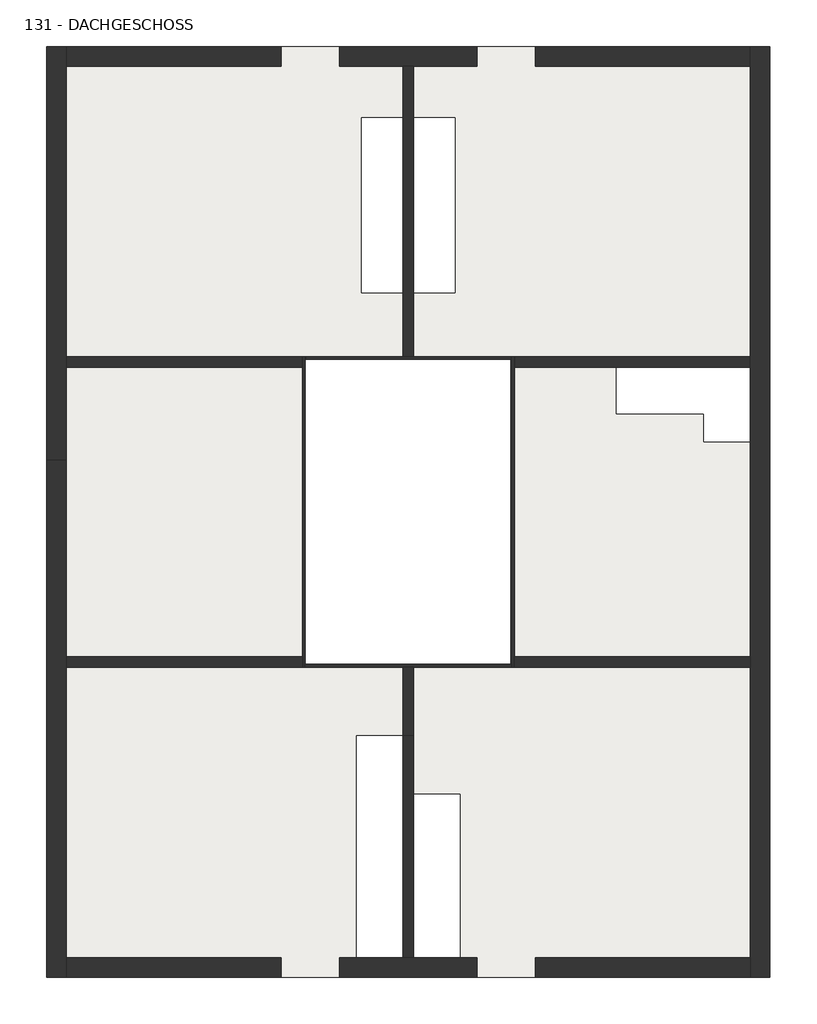
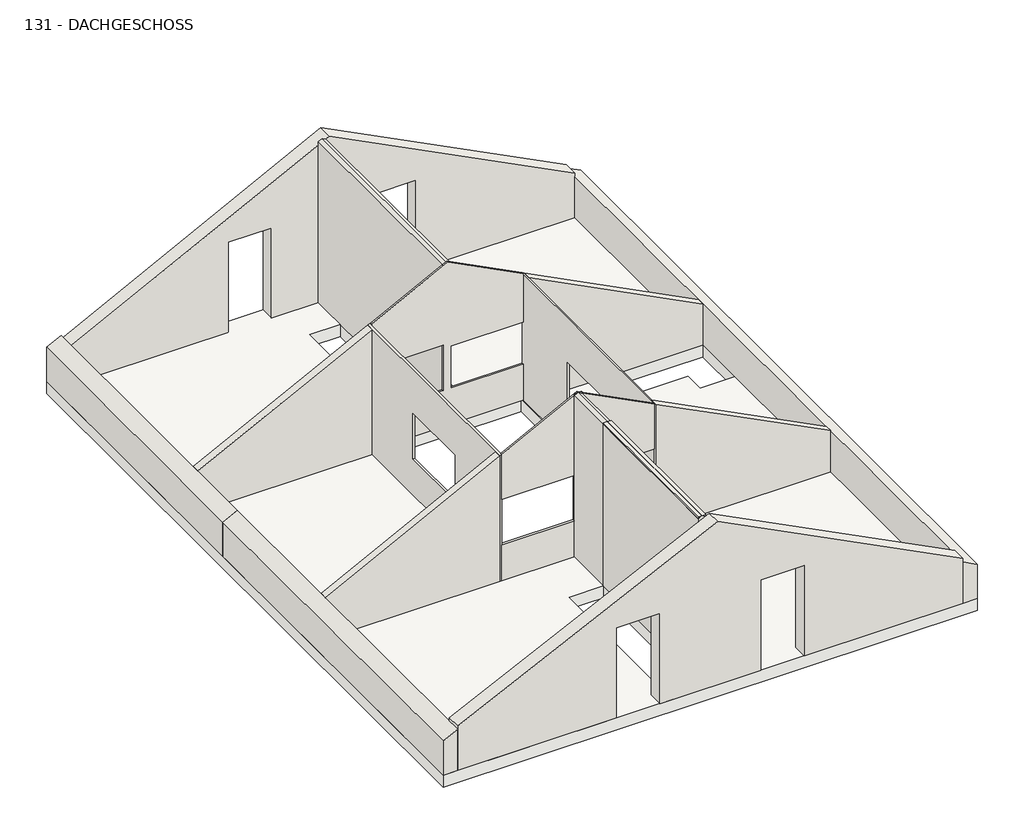
# One storey: 16 walls, 1 slab.
"""IFC4 building model written with IfcOpenShell, lengths in millimetres."""

import ifcopenshell
import ifcopenshell.guid

model = None  # the IFC model being written
_history = None  # IfcOwnerHistory: only IFC2X3 demands one
_inside = {}  # id of a spatial element -> (the spatial element, [elements in it])
_under = {}  # id of a project, library or spatial element -> (it, [spatial elements below it])
_declared = {}  # id of a project -> (the project, [libraries it declares])
_typed = {}  # id of a type object -> (the type object, [elements of that type])
_made_of = {}  # id of a material, layer set ... -> (it, [elements and type objects made of it])


def new_model(schema):
    """Start an empty IFC model of exactly this schema.

    Asked for "IFC4X3", IfcOpenShell would pick the latest addendum, in which some entities
    have other attributes; the version numbers below select the first issue.
    IFC2X3 requires an IfcOwnerHistory on every rooted entity: one is made here for all.
    """
    global model, _history
    if schema == "IFC4X3":
        model = ifcopenshell.file(schema_version=(4, 3, 0, 0))
    else:
        model = ifcopenshell.file(schema=schema)
    _inside.clear()
    _under.clear()
    _declared.clear()
    _typed.clear()
    _made_of.clear()
    _history = None
    if model.schema == "IFC2X3":
        org = make("IfcOrganization", Name="unknown")
        user = make(
            "IfcPersonAndOrganization",
            ThePerson=make("IfcPerson", FamilyName="unknown"),
            TheOrganization=org,
        )
        app = make(
            "IfcApplication",
            ApplicationDeveloper=org,
            Version="unknown",
            ApplicationFullName="unknown",
            ApplicationIdentifier="unknown",
        )
        _history = make(
            "IfcOwnerHistory",
            OwningUser=user,
            OwningApplication=app,
            ChangeAction="ADDED",
            CreationDate=0,
        )
    return model


def make(cls, **values):
    """One entity of the class cls with the attributes given. An attribute that is None is left unset."""
    return model.create_entity(
        cls, **{name: value for name, value in values.items() if value is not None}
    )


def rooted(cls, **values):
    """An entity with a GlobalId (a new one), such as an element, a storey or a relation."""
    return make(cls, GlobalId=ifcopenshell.guid.new(), OwnerHistory=_history, **values)


def si_unit(unit_type, name, prefix=None):
    """IfcSIUnit, for example si_unit("LENGTHUNIT", "METRE", prefix="MILLI")."""
    return make("IfcSIUnit", UnitType=unit_type, Prefix=prefix, Name=name)


def assignment(units):
    """IfcUnitAssignment: the units of a project."""
    return None if units is None else make("IfcUnitAssignment", Units=units)


def point(xyz):
    """IfcCartesianPoint."""
    return None if xyz is None else make("IfcCartesianPoint", Coordinates=xyz)


def direction(xyz):
    """IfcDirection."""
    return None if xyz is None else make("IfcDirection", DirectionRatios=xyz)


def frame(location, z_axis=None, x_axis=None):
    """IfcAxis2Placement3D, a coordinate frame: its origin and axes. An axis left out is left unset."""
    return make(
        "IfcAxis2Placement3D",
        Location=point(location),
        Axis=direction(z_axis),
        RefDirection=direction(x_axis),
    )


def origin():
    """The frame at (0, 0, 0) with its axes left unset."""
    return frame((0.0, 0.0, 0.0))


def place(relative_to, where):
    """IfcLocalPlacement: puts the frame where relative to a parent placement (None: the world)."""
    return make(
        "IfcLocalPlacement", PlacementRelTo=relative_to, RelativePlacement=where
    )


def context(
    kind, dimensions, precision=None, world=None, true_north=None, identifier=None
):
    """IfcGeometricRepresentationContext, for example the 3D "Model" context."""
    return make(
        "IfcGeometricRepresentationContext",
        ContextIdentifier=identifier,
        ContextType=kind,
        CoordinateSpaceDimension=dimensions,
        Precision=precision,
        WorldCoordinateSystem=world,
        TrueNorth=true_north,
    )


def project(units=None, contexts=None):
    """IfcProject with its units and contexts."""
    return rooted(
        "IfcProject",
        Name="project",
        RepresentationContexts=contexts,
        UnitsInContext=assignment(units),
    )


def spatial(cls, under=None, at=None, **own):
    """A site, building, storey or space (cls), placed at a placement, below another one or the project."""
    s = rooted(cls, ObjectPlacement=at, **own)
    if under is not None:
        _under.setdefault(under.id(), (under, []))[1].append(s)
    return s


def polyline(points):
    """IfcPolyline through the points."""
    return make("IfcPolyline", Points=[point(p) for p in points])


def outline(outer, holes=None, kind="AREA"):
    """IfcArbitraryClosedProfileDef: a profile drawn as a closed curve; with holes, ...WithVoids."""
    if holes is None:
        return make("IfcArbitraryClosedProfileDef", ProfileType=kind, OuterCurve=outer)
    return make(
        "IfcArbitraryProfileDefWithVoids",
        ProfileType=kind,
        OuterCurve=outer,
        InnerCurves=holes,
    )


def extrude(swept, where, along, depth):
    """IfcExtrudedAreaSolid: the profile swept, set in the frame where, extruded along a direction by depth."""
    return make(
        "IfcExtrudedAreaSolid",
        SweptArea=swept,
        Position=where,
        ExtrudedDirection=direction(along),
        Depth=depth,
    )


def faces_of(points, faces, orient=None, outer=None):
    """IfcFace entities. A face is a list of loops; a loop is a list of indices into points, from 0.

    orient and outer hold one flag for each loop. By default every Orientation is true, the
    first loop of a face is its IfcFaceOuterBound and the others are IfcFaceBound.
    """
    made = []
    for i, loops in enumerate(faces):
        bounds = []
        for j, loop in enumerate(loops):
            is_outer = j == 0 if outer is None else outer[i][j]
            bounds.append(
                make(
                    "IfcFaceOuterBound" if is_outer else "IfcFaceBound",
                    Bound=make("IfcPolyLoop", Polygon=[points[k] for k in loop]),
                    Orientation=True if orient is None else orient[i][j],
                )
            )
        made.append(make("IfcFace", Bounds=bounds))
    return made


def faceted_brep(points, faces, orient=None, outer=None, voids=None):
    """IfcFacetedBrep: a solid bounded by flat faces; with voids (closed shells), ...WithVoids."""
    shared = [point(p) for p in points]
    hull = make("IfcClosedShell", CfsFaces=faces_of(shared, faces, orient, outer))
    if voids is None:
        return make("IfcFacetedBrep", Outer=hull)
    return make(
        "IfcFacetedBrepWithVoids",
        Outer=hull,
        Voids=[
            make(cls, CfsFaces=faces_of(shared, fs, o, b)) for cls, fs, o, b in voids
        ],
    )


def shape(context_of_items, identifier, shape_type, items):
    """IfcShapeRepresentation: the items that make up one representation, for example the "Body"."""
    return make(
        "IfcShapeRepresentation",
        ContextOfItems=context_of_items,
        RepresentationIdentifier=identifier,
        RepresentationType=shape_type,
        Items=items,
    )


def source(mapping_origin, context_of_items, identifier, shape_type, items):
    """IfcRepresentationMap: a shape defined once, which mapped items show again and again."""
    return make(
        "IfcRepresentationMap",
        MappingOrigin=mapping_origin,
        MappedRepresentation=shape(context_of_items, identifier, shape_type, items),
    )


def transform(
    local_origin,
    x_axis=None,
    y_axis=None,
    z_axis=None,
    scale=None,
    scale2=None,
    scale3=None,
    uniform=True,
):
    """IfcCartesianTransformationOperator3D, or its non-uniform kind. x_axis, y_axis, z_axis: its Axis1, 2, 3."""
    if uniform:
        return make(
            "IfcCartesianTransformationOperator3D",
            Axis1=direction(x_axis),
            Axis2=direction(y_axis),
            LocalOrigin=point(local_origin),
            Scale=scale,
            Axis3=direction(z_axis),
        )
    return make(
        "IfcCartesianTransformationOperator3DnonUniform",
        Axis1=direction(x_axis),
        Axis2=direction(y_axis),
        LocalOrigin=point(local_origin),
        Scale=scale,
        Axis3=direction(z_axis),
        Scale2=scale2,
        Scale3=scale3,
    )


def mapped(mapping_source, mapping_target):
    """IfcMappedItem: shows the shape of a source again, moved by a transform."""
    return make(
        "IfcMappedItem", MappingSource=mapping_source, MappingTarget=mapping_target
    )


def made_of(thing, what):
    """Note that an element or type object is made of a material, layer set ...; save() writes the relation."""
    if what is not None:
        _made_of.setdefault(what.id(), (what, []))[1].append(thing)
    return thing


def element(
    cls,
    number,
    at=None,
    inside=None,
    cuts=None,
    type_object=None,
    material=None,
    context=None,
    identifier="Body",
    shape_type=None,
    held_by="IfcProductDefinitionShape",
    body=None,
    shapes=None,
    **own,
):
    """One element of the class cls, such as IfcWall. Its Tag is "e" and its number.

    at: its placement. inside: the storey or other place that contains it. cuts: it is an
    opening in that element (IfcRelVoidsElement). A single representation is given by context,
    identifier, shape_type and body (its items); several are given by shapes. held_by: the class
    of the entity that holds the representations. save() writes the other relations.
    """
    e = rooted(cls, Tag="e%d" % number, ObjectPlacement=at, **own)
    if body is not None:
        shapes = [shape(context, identifier, shape_type, body)]
    if shapes is not None:
        e.Representation = make(held_by, Representations=shapes)
    if inside is not None:
        _inside.setdefault(inside.id(), (inside, []))[1].append(e)
    if cuts is not None:
        rooted(
            "IfcRelVoidsElement", RelatingBuildingElement=cuts, RelatedOpeningElement=e
        )
    if type_object is not None:
        _typed.setdefault(type_object.id(), (type_object, []))[1].append(e)
    return made_of(e, material)


def aggregate(whole, parts):
    """IfcRelAggregates: a whole, such as a stair, and the parts it consists of."""
    return rooted("IfcRelAggregates", RelatingObject=whole, RelatedObjects=parts)


def save(model, path):
    """Write the relations noted so far, then the file.

    IfcRelAggregates (storeys below a building ...), IfcRelContainedInSpatialStructure (elements
    in a storey), IfcRelDefinesByType, IfcRelAssociatesMaterial and IfcRelDeclares: one each for
    every whole, place, type object, material and project.
    """
    for whole, parts in _under.values():
        aggregate(whole, parts)
    for where, things in _inside.values():
        rooted(
            "IfcRelContainedInSpatialStructure",
            RelatedElements=things,
            RelatingStructure=where,
        )
    for kind, things in _typed.values():
        rooted("IfcRelDefinesByType", RelatedObjects=things, RelatingType=kind)
    for what, things in _made_of.values():
        rooted("IfcRelAssociatesMaterial", RelatedObjects=things, RelatingMaterial=what)
    for by, libraries in _declared.values():
        rooted("IfcRelDeclares", RelatingContext=by, RelatedDefinitions=libraries)
    model.write(path)


def slab_52cff1b9(model_context):
    return source(origin(), model_context, "Body", "SweptSolid", [
        extrude(outline(polyline([(172797.7593015, 28481.9343946), (158797.7593015, 28481.9343946), (158797.7593015, 46484.7962965), (172797.7593015, 46484.7962965), (172797.7593015, 28481.9343946)]), holes=[polyline([(167772.7593015, 40484.7962965), (163772.7593015, 40484.7962965), (163772.7593015, 34484.7962965), (167772.7593015, 34484.7962965), (167772.7593015, 40484.7962965)]), polyline([(165697.7593015, 33159.7962965), (164797.7593015, 33159.7962965), (164797.7593015, 28861.9343946), (165697.7593015, 28861.9343946), (165697.7593015, 33159.7962965)]), polyline([(165897.7593015, 32021.9343946), (165897.7593015, 29779.7962965), (165897.7593015, 28861.9343946), (166797.7593015, 28861.9343946), (166797.7593015, 32021.9343946), (165897.7593015, 32021.9343946)]), polyline([(171517.7593015, 38844.7962965), (172417.7593015, 38844.7962965), (172417.7593015, 40284.7962965), (169822.7593015, 40284.7962965), (169822.7593015, 39384.7962965), (171517.7593015, 39384.7962965), (171517.7593015, 38844.7962965)]), polyline([(165897.7593015, 45104.7962965), (165897.7593015, 41724.7962965), (166697.7593015, 41724.7962965), (166697.7593015, 45104.7962965), (165897.7593015, 45104.7962965)]), polyline([(164897.7593015, 41724.7962965), (165697.7593015, 41724.7962965), (165697.7593015, 45104.7962965), (164897.7593015, 45104.7962965), (164897.7593015, 41724.7962965)])]), frame((0.0, 0.0, 5830.0), z_axis=(0.0, 0.0, 1.0), x_axis=(1.0, 0.0, 0.0)), (0.0, 0.0, 1.0), 330.0),
    ])


model = new_model("IFC4")

# Units and contexts
model_context = context("Model", 3, world=origin())
ifc_project = project(units=[si_unit("LENGTHUNIT", "METRE", prefix="MILLI")], contexts=[model_context])

# Site, building, storey
site = spatial("IfcSite", under=ifc_project)
building = spatial("IfcBuilding", under=site)
storey = spatial("IfcBuildingStorey", under=building, Name="131 - DACHGESCHOSS", Elevation=5650.0)

# Slab
placement = place(None, origin())
slab_shape = slab_52cff1b9(model_context)
element("IfcSlab", 1, ObjectType="Holzdecke 142136 : Holzdecke 142136", at=placement, inside=storey, context=model_context, shape_type="MappedRepresentation", body=[
    mapped(slab_shape, transform((-157297.7593015, -26934.7962965, 0.0), x_axis=(1.0, 0.0, 0.0), y_axis=(0.0, 1.0, 0.0), z_axis=(0.0, 0.0, 1.0))),
])

# Walls
element("IfcWall", 2, ObjectType="Holzwand", at=placement, inside=storey, context=model_context, shape_type="SweptSolid", body=[
    extrude(outline(polyline([(6160.0, 10550.0), (6160.0, 15120.0), (7303.6196708, 15120.0), (9632.150975, 10550.0), (6160.0, 10550.0)])), frame((0.0, 7550.0, 0.0), z_axis=(0.0, 1.0, 0.0), x_axis=(0.0, 0.0, 1.0)), (0.0, 0.0, 1.0), 200.0),
])
element("IfcWall", 3, ObjectType="Holzwand:1197", at=placement, inside=storey, context=model_context, shape_type="SweptSolid", body=[
    extrude(outline(polyline([(6160.0, 1880.0), (6160.0, 6450.0), (9632.150975, 6450.0), (7303.6196708, 1880.0), (6160.0, 1880.0)])), frame((0.0, 7550.0, 0.0), z_axis=(0.0, 1.0, 0.0), x_axis=(0.0, 0.0, 1.0)), (0.0, 0.0, 1.0), 200.0),
])
element("IfcWall", 4, ObjectType="Holzwand:1195", at=placement, inside=storey, context=model_context, shape_type="SweptSolid", body=[
    extrude(outline(polyline([(6160.0, 10550.0), (6160.0, 15120.0), (7303.6196708, 15120.0), (9632.150975, 10550.0), (6160.0, 10550.0)])), frame((0.0, 13350.0, 0.0), z_axis=(0.0, 1.0, 0.0), x_axis=(0.0, 0.0, 1.0)), (0.0, 0.0, 1.0), 200.0),
])
element("IfcWall", 5, ObjectType="Holzwand:1193", at=placement, inside=storey, context=model_context, shape_type="SweptSolid", body=[
    extrude(outline(polyline([(6160.0, 1880.0), (6160.0, 6450.0), (9632.150975, 6450.0), (7303.6196708, 1880.0), (6160.0, 1880.0)])), frame((0.0, 13350.0, 0.0), z_axis=(0.0, 1.0, 0.0), x_axis=(0.0, 0.0, 1.0)), (0.0, 0.0, 1.0), 200.0),
])
element("IfcWall", 6, ObjectType=" ", at=placement, inside=storey, context=model_context, shape_type="Brep", body=[
    faceted_brep([(6500.0, 7550.0, 6160.0), (6500.0, 7600.0, 6160.0), (6500.0, 13550.0, 6160.0), (6500.0, 13550.0, 9657.6272475), (6500.0, 7600.0, 9657.6272475), (6500.0, 7550.0, 9657.6272475), (6500.0, 7550.0, 8420.0), (6500.0, 7550.0, 7160.0), (6500.0, 11500.0, 8420.0), (6500.0, 11500.0, 7160.0), (6500.0, 9600.0, 7160.0), (6500.0, 9600.0, 8420.0), (6450.0, 13550.0, 6160.0), (6450.0, 7550.0, 6160.0), (6450.0, 7550.0, 9632.150975), (6450.0, 13550.0, 9632.150975), (6450.0, 11500.0, 7160.0), (6450.0, 11500.0, 8420.0), (6450.0, 9600.0, 8420.0), (6450.0, 9600.0, 7160.0)], [[[0, 1, 2, 3, 4, 5, 6, 7], [8, 9, 10, 11]], [[12, 13, 14, 15], [16, 17, 18, 19]], [[2, 1, 0, 13, 12]], [[5, 4, 3, 15, 14]], [[8, 17, 16, 9]], [[17, 8, 11, 18]], [[18, 11, 10, 19]], [[9, 16, 19, 10]], [[0, 7, 6, 5, 14, 13]], [[3, 2, 12, 15]]]),
])
element("IfcWall", 7, ObjectType=" :1188", at=placement, inside=storey, context=model_context, shape_type="Brep", body=[
    faceted_brep([(10500.0, 7600.0, 6160.0), (6500.0, 7600.0, 6160.0), (6500.0, 7600.0, 7160.0), (8400.0, 7600.0, 7160.0), (8400.0, 7600.0, 8420.0), (6500.0, 7600.0, 8420.0), (6500.0, 7600.0, 9657.6272475), (8500.0, 7600.0, 10676.6781465), (10500.0, 7600.0, 9657.6272475), (10500.0, 7600.0, 8420.0), (8607.9636779, 7600.0, 8420.0), (8607.9636779, 7600.0, 7160.0), (10500.0, 7600.0, 7160.0), (6500.0, 7550.0, 6160.0), (10500.0, 7550.0, 6160.0), (10500.0, 7550.0, 7160.0), (8607.9636779, 7550.0, 7160.0), (8607.9636779, 7550.0, 8420.0), (10500.0, 7550.0, 8420.0), (10500.0, 7550.0, 9657.6272475), (8600.0, 7550.0, 10625.7256015), (8600.0, 7550.0, 10676.6781465), (8400.0, 7550.0, 10676.6781465), (8400.0, 7550.0, 10625.7256015), (6500.0, 7550.0, 9657.6272475), (6500.0, 7550.0, 8420.0), (8400.0, 7550.0, 8420.0), (8400.0, 7550.0, 7160.0), (6500.0, 7550.0, 7160.0), (8500.0, 7550.4030929, 10676.6781465)], [[[0, 1, 2, 3, 4, 5, 6, 7, 8, 9, 10, 11, 12]], [[13, 14, 15, 16, 17, 18, 19, 20, 21, 22, 23, 24, 25, 26, 27, 28]], [[1, 0, 14, 13]], [[22, 21, 29]], [[29, 20, 19, 8, 7]], [[20, 29, 21]], [[29, 7, 6, 24, 23]], [[29, 23, 22]], [[4, 26, 25, 5]], [[26, 4, 3, 27]], [[27, 3, 2, 28]], [[10, 17, 16, 11]], [[17, 10, 9, 18]], [[11, 16, 15, 12]], [[8, 19, 18, 9]], [[14, 0, 12, 15]], [[24, 6, 5, 25]], [[1, 13, 28, 2]]]),
])
element("IfcWall", 8, ObjectType=" :1186", at=placement, inside=storey, context=model_context, shape_type="Brep", body=[
    faceted_brep([(10500.0, 13550.0, 6160.0), (10500.0, 13500.0, 6160.0), (10500.0, 7600.0, 6160.0), (10500.0, 7550.0, 6160.0), (10500.0, 7550.0, 7160.0), (10500.0, 7550.0, 8420.0), (10500.0, 7550.0, 9657.6272475), (10500.0, 7600.0, 9657.6272475), (10500.0, 13550.0, 9657.6272475), (10500.0, 13550.0, 8320.0), (10500.0, 13550.0, 7160.0), (10500.0, 9600.0, 8420.0), (10500.0, 9600.0, 7160.0), (10500.0, 11500.0, 7160.0), (10500.0, 11500.0, 8420.0), (10550.0, 7550.0, 6160.0), (10550.0, 13550.0, 6160.0), (10550.0, 13550.0, 9632.150975), (10550.0, 7550.0, 9632.150975), (10550.0, 9600.0, 7160.0), (10550.0, 9600.0, 8420.0), (10550.0, 11500.0, 8420.0), (10550.0, 11500.0, 7160.0)], [[[0, 1, 2, 3, 4, 5, 6, 7, 8, 9, 10], [11, 12, 13, 14]], [[15, 16, 17, 18], [19, 20, 21, 22]], [[3, 2, 1, 0, 16, 15]], [[8, 7, 6, 18, 17]], [[19, 12, 11, 20]], [[20, 11, 14, 21]], [[21, 14, 13, 22]], [[12, 19, 22, 13]], [[6, 5, 4, 3, 15, 18]], [[0, 10, 9, 8, 17, 16]]]),
])
element("IfcWall", 9, ObjectType="Holzwand:1184", at=placement, inside=storey, context=model_context, shape_type="SweptSolid", body=[
    extrude(outline(polyline([(6160.0, 8400.0), (6160.0, 8600.0), (10625.7256015, 8600.0), (10676.6781465, 8500.0), (10625.7256015, 8400.0), (6160.0, 8400.0)])), frame((0.0, 1927.1380981, 0.0), z_axis=(0.0, 1.0, 0.0), x_axis=(0.0, 0.0, 1.0)), (0.0, 0.0, 1.0), 4297.8619019),
])
element("IfcWall", 10, ObjectType="Holzwand:1180", at=placement, inside=storey, context=model_context, shape_type="SweptSolid", body=[
    extrude(outline(polyline([(6160.0, 8400.0), (6160.0, 8600.0), (10625.7256015, 8600.0), (10676.6781465, 8500.0), (10625.7256015, 8400.0), (6160.0, 8400.0)])), frame((0.0, 13550.0, 0.0), z_axis=(0.0, 1.0, 0.0), x_axis=(0.0, 0.0, 1.0)), (0.0, 0.0, 1.0), 5620.0),
])
element("IfcWall", 11, ObjectType="Holzwand:1178", at=placement, inside=storey, context=model_context, shape_type="Brep", body=[
    faceted_brep([(8600.0, 1927.541191, 6160.0), (8600.0, 7550.0, 6160.0), (8600.0, 7550.0, 10625.7256015), (8600.0, 6225.0, 10625.7256015), (8600.0, 6225.0, 10676.6781465), (8600.0, 1927.541191, 10676.6781465), (8400.0, 7550.0, 6160.0), (8400.0, 1927.541191, 6160.0), (8400.0, 1927.541191, 10676.6781465), (8400.0, 6225.0, 10676.6781465), (8400.0, 6225.0, 10625.7256015), (8400.0, 7550.0, 10625.7256015), (8500.0, 6225.0, 10676.6781465), (8500.0, 7550.0, 10676.6781465)], [[[0, 1, 2, 3, 4, 5]], [[6, 7, 8, 9, 10, 11]], [[1, 0, 7, 6]], [[8, 5, 4, 12, 9]], [[0, 5, 8, 7]], [[12, 3, 2, 13]], [[3, 12, 4]], [[12, 10, 9]], [[10, 12, 13, 11]], [[1, 6, 11, 13, 2]]]),
])
element("IfcWall", 12, ObjectType=" :1190", at=placement, inside=storey, context=model_context, shape_type="Brep", body=[
    faceted_brep([(6525.0, 13500.0, 6160.0), (10500.0, 13500.0, 6160.0), (10500.0, 13500.0, 7160.0), (8600.0, 13500.0, 7160.0), (8600.0, 13500.0, 8320.0), (10500.0, 13500.0, 8320.0), (10500.0, 13500.0, 9670.3653837), (8525.0, 13500.0, 10676.6781465), (6525.0, 13500.0, 9657.6272475), (6525.0, 13500.0, 8420.0), (8400.0, 13500.0, 8420.0), (8400.0, 13500.0, 7160.0), (6525.0, 13500.0, 7160.0), (10500.0, 13550.0, 6160.0), (6525.0, 13550.0, 6160.0), (6525.0, 13550.0, 7160.0), (8400.0, 13550.0, 7160.0), (8400.0, 13550.0, 8420.0), (6525.0, 13550.0, 8420.0), (6525.0, 13550.0, 9657.6272475), (8525.0, 13550.0, 10676.6781465), (10500.0, 13550.0, 9670.3653837), (10500.0, 13550.0, 9657.6272475), (10500.0, 13550.0, 8320.0), (8600.0, 13550.0, 8320.0), (8600.0, 13550.0, 7160.0), (10500.0, 13550.0, 7160.0)], [[[0, 1, 2, 3, 4, 5, 6, 7, 8, 9, 10, 11, 12]], [[13, 14, 15, 16, 17, 18, 19, 20, 21, 22, 23, 24, 25, 26]], [[1, 0, 14, 13]], [[7, 6, 21, 20]], [[8, 7, 20, 19]], [[8, 19, 18, 9]], [[14, 0, 12, 15]], [[10, 17, 16, 11]], [[17, 10, 9, 18]], [[11, 16, 15, 12]], [[4, 24, 23, 5]], [[24, 4, 3, 25]], [[25, 3, 2, 26]], [[21, 6, 5, 23, 22]], [[1, 13, 26, 2]]]),
])
element("IfcWall", 13, ObjectType="1141 Aussenwand", at=placement, inside=storey, context=model_context, shape_type="Brep", body=[
    faceted_brep([(1880.0, 1547.1380981, 6160.0), (1880.0, 1927.1380981, 6160.0), (1880.0, 11550.0, 6160.0), (1880.0, 11550.0, 7303.6196708), (1880.0, 1547.1380981, 7303.6196708), (1500.0, 11550.0, 6160.0), (1500.0, 1547.1380981, 6160.0), (1500.0, 1547.1380981, 7110.0), (1500.0, 11550.0, 7110.0)], [[[0, 1, 2, 3, 4]], [[5, 6, 7, 8]], [[2, 1, 0, 6, 5]], [[3, 2, 5, 8]], [[4, 3, 8, 7]], [[0, 4, 7, 6]]]),
])
element("IfcWall", 14, ObjectType="1141 Aussenwand", at=placement, inside=storey, context=model_context, shape_type="Brep", body=[
    faceted_brep([(15120.0, 19550.0, 6160.0), (15120.0, 19170.0, 6160.0), (15120.0, 1927.1380981, 6160.0), (15120.0, 1547.1380981, 6160.0), (15120.0, 1547.1380981, 7303.6196708), (15120.0, 19550.0, 7303.6196708), (15500.0, 1547.1380981, 6160.0), (15500.0, 19550.0, 6160.0), (15500.0, 19550.0, 7110.0), (15500.0, 1547.1380981, 7110.0)], [[[0, 1, 2, 3, 4, 5]], [[6, 7, 8, 9]], [[3, 2, 1, 0, 7, 6]], [[5, 4, 9, 8]], [[4, 3, 6, 9]], [[0, 5, 8, 7]]]),
])
element("IfcWall", 15, ObjectType="1141 Aussenwand", at=placement, inside=storey, context=model_context, shape_type="Brep", body=[
    faceted_brep([(1880.0, 11550.0, 6160.0), (1880.0, 19170.0, 6160.0), (1880.0, 19550.0, 6160.0), (1880.0, 19550.0, 7206.8098354), (1880.0, 19550.0, 7303.6196708), (1880.0, 11550.0, 7303.6196708), (1500.0, 19550.0, 6160.0), (1500.0, 11550.0, 6160.0), (1500.0, 11550.0, 7110.0), (1500.0, 19550.0, 7110.0)], [[[0, 1, 2, 3, 4, 5]], [[6, 7, 8, 9]], [[2, 1, 0, 7, 6]], [[0, 5, 8, 7]], [[5, 4, 9, 8]], [[4, 3, 2, 6, 9]]]),
])
element("IfcWall", 16, ObjectType="1141 Aussenwand", at=placement, inside=storey, context=model_context, shape_type="Brep", body=[
    faceted_brep([(1880.0, 1927.1380981, 7395.1741151), (8690.0, 1927.1380981, 10676.6781465), (15120.0, 1927.1380981, 7400.4295062), (15120.0, 1927.1380981, 6160.0), (10960.0, 1927.1380981, 6160.0), (10960.0, 1927.1380981, 8660.0), (9825.0, 1927.1380981, 8660.0), (9825.0, 1927.1380981, 6160.0), (7175.0, 1927.1380981, 6160.0), (7175.0, 1927.1380981, 8660.0), (6040.0, 1927.1380981, 8660.0), (6040.0, 1927.1380981, 6160.0), (1880.0, 1927.1380981, 6160.0), (8690.0, 1547.1380981, 10676.6781465), (1880.0, 1547.1380981, 7395.1741151), (1880.0, 1547.1380981, 7303.6196708), (1880.0, 1547.1380981, 6160.0), (6040.0, 1547.1380981, 6160.0), (6040.0, 1547.1380981, 8660.0), (7175.0, 1547.1380981, 8660.0), (7175.0, 1547.1380981, 6160.0), (9825.0, 1547.1380981, 6160.0), (9825.0, 1547.1380981, 8660.0), (10960.0, 1547.1380981, 8660.0), (10960.0, 1547.1380981, 6160.0), (15120.0, 1547.1380981, 6160.0), (15120.0, 1547.1380981, 7303.6196708), (15120.0, 1547.1380981, 7400.4295062)], [[[0, 1, 2, 3, 4, 5, 6, 7, 8, 9, 10, 11, 12]], [[13, 14, 15, 16, 17, 18, 19, 20, 21, 22, 23, 24, 25, 26, 27]], [[4, 3, 25, 24]], [[7, 21, 20, 8]], [[16, 12, 11, 17]], [[1, 0, 14, 13]], [[2, 1, 13, 27]], [[23, 5, 4, 24]], [[5, 23, 22, 6]], [[6, 22, 21, 7]], [[19, 9, 8, 20]], [[9, 19, 18, 10]], [[10, 18, 17, 11]], [[0, 12, 16, 15, 14]], [[3, 2, 27, 26, 25]]]),
])
element("IfcWall", 17, ObjectType="1141 Aussenwand", at=placement, inside=storey, context=model_context, shape_type="Brep", body=[
    faceted_brep([(15120.0, 19170.0, 7400.4295062), (8690.0, 19170.0, 10676.6781465), (1880.0, 19170.0, 7206.8098354), (1880.0, 19170.0, 6160.0), (6040.0, 19170.0, 6160.0), (6040.0, 19170.0, 8660.0), (7175.0, 19170.0, 8660.0), (7175.0, 19170.0, 6160.0), (9825.0, 19170.0, 6160.0), (9825.0, 19170.0, 8660.0), (10960.0, 19170.0, 8660.0), (10960.0, 19170.0, 6160.0), (15120.0, 19170.0, 6160.0), (8690.0, 19550.0, 10676.6781465), (15120.0, 19550.0, 7400.4295062), (15120.0, 19550.0, 7303.6196708), (15120.0, 19550.0, 6160.0), (10960.0, 19550.0, 6160.0), (10960.0, 19550.0, 8660.0), (9825.0, 19550.0, 8660.0), (9825.0, 19550.0, 6160.0), (7175.0, 19550.0, 6160.0), (7175.0, 19550.0, 8660.0), (6040.0, 19550.0, 8660.0), (6040.0, 19550.0, 6160.0), (1880.0, 19550.0, 6160.0), (1880.0, 19550.0, 7206.8098354)], [[[0, 1, 2, 3, 4, 5, 6, 7, 8, 9, 10, 11, 12]], [[13, 14, 15, 16, 17, 18, 19, 20, 21, 22, 23, 24, 25, 26]], [[12, 11, 17, 16]], [[20, 8, 7, 21]], [[3, 25, 24, 4]], [[1, 0, 14, 13]], [[2, 1, 13, 26]], [[19, 9, 8, 20]], [[9, 19, 18, 10]], [[10, 18, 17, 11]], [[23, 5, 4, 24]], [[5, 23, 22, 6]], [[6, 22, 21, 7]], [[0, 12, 16, 15, 14]], [[3, 2, 26, 25]]]),
])

save(model, "model.ifc")

# Revit data of these elements
# Type "Holzdecke 142136 : Holzdecke 142136"
#   Abrechnungsart = "m²"
#   Allright_Bauteil_ID = "0123De 0783954319"
#   Bezeichnung = "Holzdecke"
#   Codetext = "D-HOLZBALKEN1\\"
#   Gewerk = "Zimmer- und Holzbauarbeiten"
#   Material = "Holz"
#   Objektname = "Brettstapeldecke"
#   NameOverride = "Holzdecke"
#   Reference = "Holzdecke"
#   Status = "NEW"
#   PitchAngle = 0.00°
#   ThermalTransmittance = 0.0000 BTU/(h·ft²·°F)
#   2D Interaktion = yes
#   Combustible = no
#   Compartmentation = no
#   IsExternal = no
#   LoadBearing = yes
# Type "Holzwand"
#   ThermalTransmittance = 0.0000 BTU/(h·ft²·°F)
#   Combustible = no
#   Compartmentation = no
#   Layers, outside or top first: 0.200 m "holzschalung" (function 1)
# Type "Holzwand:1197"
#   ThermalTransmittance = 0.0000 BTU/(h·ft²·°F)
#   Combustible = no
#   Compartmentation = no
#   Layers, outside or top first: 0.200 m "holzschalung" (function 1)
# Type "Holzwand:1195"
#   ThermalTransmittance = 0.0000 BTU/(h·ft²·°F)
#   Combustible = no
#   Compartmentation = no
#   Layers, outside or top first: 0.200 m "holzschalung" (function 1)
# Type "Holzwand:1193"
#   ThermalTransmittance = 0.0000 BTU/(h·ft²·°F)
#   Combustible = no
#   Compartmentation = no
#   Layers, outside or top first: 0.200 m "holzschalung" (function 1)
# Type " "
#   Layers, outside or top first: 0.050 m "holzschalung" (function 1)
# Type " :1188"
#   Layers, outside or top first: 0.050 m "holzschalung" (function 1)
# Type " :1186"
#   Layers, outside or top first: 0.050 m "holzschalung" (function 1)
# Type "Holzwand:1184"
#   ThermalTransmittance = 0.0000 BTU/(h·ft²·°F)
#   Combustible = no
#   Compartmentation = no
#   Layers, outside or top first: 0.200 m "holzschalung" (function 1)
# Type "Holzwand:1180"
#   ThermalTransmittance = 0.0000 BTU/(h·ft²·°F)
#   Combustible = no
#   Compartmentation = no
#   Layers, outside or top first: 0.200 m "holzschalung" (function 1)
# Type "Holzwand:1178"
#   ThermalTransmittance = 0.0000 BTU/(h·ft²·°F)
#   Combustible = no
#   Compartmentation = no
#   Layers, outside or top first: 0.200 m "holzschalung" (function 1)
# Type " :1190"
#   Layers, outside or top first: 0.050 m "holzschalung" (function 1)
# Type "1141 Aussenwand"
#   Layers, outside or top first: 0.380 m "holzschalung" (function 1)
# Element 1 (IfcSlab, "Holzdecke 142136 : Holzdecke 142136")
#   IFC Predefined Type = "FLOOR"
#   Export to IFC As = "ifcslab"
#   IfcGUID = "2UFX_hum15ZQP8rfQ2hTBa"
#   Phase Created = New Construction
#   Materials on its faces: "holzschalung"
# Element 2 (IfcWall, "Holzwand")
#   Export to IFC As = "ifcwall"
#   IfcGUID = "2irPo0fN95hwd6nGWO8xKX"
#   NameOverride = "Holzwand"
#   Abrechnungsart = "St"
#   Allright_Bauteil_ID = "0131HWa0658953274"
#   Bezeichnung = "Holzwand"
#   Layer #1:Object Layer Attributes #1:Abrechnungsart = "m²"
#   Layer #1:Object Layer Attributes #1:Allright_Bauteil_ID = "0131Wa 0658953275"
#   Layer #1:Object Layer Attributes #1:Bezeichnung = "Holzwand"
#   Layer #1:Object Layer Attributes #1:Codetext = "HO-WI-HSW\\"
#   Layer #1:Object Layer Attributes #1:Gewerk = "Zimmer- und Holzbauarbeiten"
#   Layer #1:Object Layer Attributes #1:Material = "Holz"
#   Layer #1:Object Layer Attributes #1:Objektname = "Wand"
#   Layer #1:Object Layer Attributes #1:Reference = "Holzwand"
#   Layer #1:Object Layer Attributes #1:Status = "Neubau"
#   MEP Wandtyp = "HO-WA-HSW\\"
#   Objektname = "Gesamtwand"
#   Reference = "Holzwand"
#   Status = "NEW"
#   built-in parameter 1001111 = 0.510 m
#   Top Offset = 0.000 m
#   Base Offset = 0.510 m
#   Unconnected Height = 3.497627 m
#   wall height = 3.497627 m
#   Layer #1:Object Layer Attributes #1:U-Wert = 0
#   Layer #1:Object Layer Attributes #1:2D Interaktion = yes
#   Layer #1:Object Layer Attributes #1:Außenbauteil = no
#   Layer #1:Object Layer Attributes #1:Brandabschnittsdefinierendes Bauteil = no
#   Layer #1:Object Layer Attributes #1:Brennbares Material = no
#   Layer #1:Object Layer Attributes #1:Raumhohe Wand = yes
#   Layer #1:Object Layer Attributes #1:Tragendes Bauteil = yes
#   ExtendToStructure = yes
#   IsExternal = no
#   LoadBearing = yes
#   Phase Created = New Construction
#   Base Constraint = 131 - DACHGESCHOSS
#   Materials on its faces: "holzschalung"
# Element 3 (IfcWall, "Holzwand:1197")
#   Export to IFC As = "ifcwall"
#   IfcGUID = "0btdfUgAf1BODjBN4XyqI6"
#   NameOverride = "Holzwand"
#   Abrechnungsart = "St"
#   Allright_Bauteil_ID = "0131HWa0658955859"
#   Bezeichnung = "Holzwand"
#   Layer #1:Object Layer Attributes #1:Abrechnungsart = "m²"
#   Layer #1:Object Layer Attributes #1:Allright_Bauteil_ID = "0131Wa 0658955860"
#   Layer #1:Object Layer Attributes #1:Bezeichnung = "Holzwand"
#   Layer #1:Object Layer Attributes #1:Codetext = "HO-WI-HSW\\"
#   Layer #1:Object Layer Attributes #1:Gewerk = "Zimmer- und Holzbauarbeiten"
#   Layer #1:Object Layer Attributes #1:Material = "Holz"
#   Layer #1:Object Layer Attributes #1:Objektname = "Wand"
#   Layer #1:Object Layer Attributes #1:Reference = "Holzwand"
#   Layer #1:Object Layer Attributes #1:Status = "Neubau"
#   MEP Wandtyp = "HO-WA-HSW\\"
#   Objektname = "Gesamtwand"
#   Reference = "Holzwand"
#   Status = "NEW"
#   built-in parameter 1001111 = 0.510 m
#   Top Offset = 0.000 m
#   Base Offset = 0.510 m
#   Unconnected Height = 3.497627 m
#   wall height = 3.497627 m
#   Layer #1:Object Layer Attributes #1:U-Wert = 0
#   Layer #1:Object Layer Attributes #1:2D Interaktion = yes
#   Layer #1:Object Layer Attributes #1:Außenbauteil = no
#   Layer #1:Object Layer Attributes #1:Brandabschnittsdefinierendes Bauteil = no
#   Layer #1:Object Layer Attributes #1:Brennbares Material = no
#   Layer #1:Object Layer Attributes #1:Raumhohe Wand = yes
#   Layer #1:Object Layer Attributes #1:Tragendes Bauteil = yes
#   ExtendToStructure = yes
#   IsExternal = no
#   LoadBearing = yes
#   Phase Created = New Construction
#   Base Constraint = 131 - DACHGESCHOSS
#   Materials on its faces: "holzschalung"
# Element 4 (IfcWall, "Holzwand:1195")
#   Export to IFC As = "ifcwall"
#   IfcGUID = "2RQ2xt8jL3z9U7Ow04WNfJ"
#   NameOverride = "Holzwand"
#   Abrechnungsart = "St"
#   Allright_Bauteil_ID = "0131HWa0658953259"
#   Bezeichnung = "Holzwand"
#   Layer #1:Object Layer Attributes #1:Abrechnungsart = "m²"
#   Layer #1:Object Layer Attributes #1:Allright_Bauteil_ID = "0131Wa 0658953260"
#   Layer #1:Object Layer Attributes #1:Bezeichnung = "Holzwand"
#   Layer #1:Object Layer Attributes #1:Codetext = "HO-WI-HSW\\"
#   Layer #1:Object Layer Attributes #1:Gewerk = "Zimmer- und Holzbauarbeiten"
#   Layer #1:Object Layer Attributes #1:Material = "Holz"
#   Layer #1:Object Layer Attributes #1:Objektname = "Wand"
#   Layer #1:Object Layer Attributes #1:Reference = "Holzwand"
#   Layer #1:Object Layer Attributes #1:Status = "Neubau"
#   MEP Wandtyp = "HO-WA-HSW\\"
#   Objektname = "Gesamtwand"
#   Reference = "Holzwand"
#   Status = "NEW"
#   built-in parameter 1001111 = 0.510 m
#   Top Offset = 0.000 m
#   Base Offset = 0.510 m
#   Unconnected Height = 3.497627 m
#   wall height = 3.497627 m
#   Layer #1:Object Layer Attributes #1:U-Wert = 0
#   Layer #1:Object Layer Attributes #1:2D Interaktion = yes
#   Layer #1:Object Layer Attributes #1:Außenbauteil = no
#   Layer #1:Object Layer Attributes #1:Brandabschnittsdefinierendes Bauteil = no
#   Layer #1:Object Layer Attributes #1:Brennbares Material = no
#   Layer #1:Object Layer Attributes #1:Raumhohe Wand = yes
#   Layer #1:Object Layer Attributes #1:Tragendes Bauteil = yes
#   ExtendToStructure = yes
#   IsExternal = no
#   LoadBearing = yes
#   Phase Created = New Construction
#   Base Constraint = 131 - DACHGESCHOSS
#   Materials on its faces: "holzschalung"
# Element 5 (IfcWall, "Holzwand:1193")
#   Export to IFC As = "ifcwall"
#   IfcGUID = "1XDlXo4IT97OvdyoFppHWZ"
#   NameOverride = "Holzwand"
#   Abrechnungsart = "St"
#   Allright_Bauteil_ID = "0131HWa0658952486"
#   Bezeichnung = "Holzwand"
#   Layer #1:Object Layer Attributes #1:Abrechnungsart = "m²"
#   Layer #1:Object Layer Attributes #1:Allright_Bauteil_ID = "0131Wa 0658952490"
#   Layer #1:Object Layer Attributes #1:Bezeichnung = "Holzwand"
#   Layer #1:Object Layer Attributes #1:Codetext = "HO-WI-HSW\\"
#   Layer #1:Object Layer Attributes #1:Gewerk = "Zimmer- und Holzbauarbeiten"
#   Layer #1:Object Layer Attributes #1:Material = "Holz"
#   Layer #1:Object Layer Attributes #1:Objektname = "Wand"
#   Layer #1:Object Layer Attributes #1:Reference = "Holzwand"
#   Layer #1:Object Layer Attributes #1:Status = "Neubau"
#   MEP Wandtyp = "HO-WA-HSW\\"
#   Objektname = "Gesamtwand"
#   Reference = "Holzwand"
#   Status = "NEW"
#   built-in parameter 1001111 = 0.510 m
#   Top Offset = 0.000 m
#   Base Offset = 0.510 m
#   Unconnected Height = 3.497627 m
#   wall height = 3.497627 m
#   Layer #1:Object Layer Attributes #1:U-Wert = 0
#   Layer #1:Object Layer Attributes #1:2D Interaktion = yes
#   Layer #1:Object Layer Attributes #1:Außenbauteil = no
#   Layer #1:Object Layer Attributes #1:Brandabschnittsdefinierendes Bauteil = no
#   Layer #1:Object Layer Attributes #1:Brennbares Material = no
#   Layer #1:Object Layer Attributes #1:Raumhohe Wand = yes
#   Layer #1:Object Layer Attributes #1:Tragendes Bauteil = yes
#   ExtendToStructure = yes
#   IsExternal = no
#   LoadBearing = yes
#   Phase Created = New Construction
#   Base Constraint = 131 - DACHGESCHOSS
#   Materials on its faces: "holzschalung"
# Element 6 (IfcWall, " ")
#   Export to IFC As = "ifcwall"
#   IfcGUID = "21FF_DgHzF28s1dzPXnAcl"
#   NameOverride = " "
#   Abrechnungsart = "m³"
#   Allright_Bauteil_ID = "0131HWa0658952409"
#   Layer #1:Object Layer Attributes #1:Abrechnungsart = "m²"
#   Layer #1:Object Layer Attributes #1:Allright_Bauteil_ID = "0131Wa 0658952493"
#   Layer #1:Object Layer Attributes #1:Gewerk = "Zimmer- und Holzbauarbeiten"
#   Layer #1:Object Layer Attributes #1:Material = "k.Ausw."
#   Layer #1:Object Layer Attributes #1:Objektname = "Wand"
#   Layer #1:Object Layer Attributes #1:Status = "Neubau"
#   MEP Wandtyp = "HO-WA-HSW\\"
#   Objektname = "Gesamtwand"
#   built-in parameter 1001111 = 0.510 m
#   Top Offset = 0.000 m
#   Base Offset = 0.510 m
#   Unconnected Height = 3.497627 m
#   wall height = 3.497627 m
#   Layer #1:Object Layer Attributes #1:2D Interaktion = yes
#   Phase Created = New Construction
#   Base Constraint = 131 - DACHGESCHOSS
#   Materials on its faces: "holzschalung"
# Element 7 (IfcWall, " :1188")
#   Export to IFC As = "ifcwall"
#   IfcGUID = "1sDERupobB$8G6O8zmS_FC"
#   NameOverride = " "
#   Abrechnungsart = "m³"
#   Allright_Bauteil_ID = "0131HWa0658952407"
#   Layer #1:Object Layer Attributes #1:Abrechnungsart = "m²"
#   Layer #1:Object Layer Attributes #1:Allright_Bauteil_ID = "0131Wa 0658952497"
#   Layer #1:Object Layer Attributes #1:Gewerk = "Zimmer- und Holzbauarbeiten"
#   Layer #1:Object Layer Attributes #1:Material = "k.Ausw."
#   Layer #1:Object Layer Attributes #1:Objektname = "Wand"
#   Layer #1:Object Layer Attributes #1:Status = "Neubau"
#   MEP Wandtyp = "HO-WA-HSW\\"
#   Objektname = "Gesamtwand"
#   built-in parameter 1001111 = 0.510 m
#   Top Offset = 0.000 m
#   Base Offset = 0.510 m
#   Unconnected Height = 4.516678 m
#   wall height = 4.516678 m
#   Layer #1:Object Layer Attributes #1:2D Interaktion = yes
#   Phase Created = New Construction
#   Base Constraint = 131 - DACHGESCHOSS
#   Materials on its faces: "holzschalung"
# Element 8 (IfcWall, " :1186")
#   Export to IFC As = "ifcwall"
#   IfcGUID = "2vPa_8WInC1fLjRjt9C8qD"
#   NameOverride = " "
#   Abrechnungsart = "m³"
#   Allright_Bauteil_ID = "0131HWa0658952411"
#   Layer #1:Object Layer Attributes #1:Abrechnungsart = "m²"
#   Layer #1:Object Layer Attributes #1:Allright_Bauteil_ID = "0131Wa 0658952482"
#   Layer #1:Object Layer Attributes #1:Gewerk = "Zimmer- und Holzbauarbeiten"
#   Layer #1:Object Layer Attributes #1:Material = "k.Ausw."
#   Layer #1:Object Layer Attributes #1:Objektname = "Wand"
#   Layer #1:Object Layer Attributes #1:Status = "Neubau"
#   MEP Wandtyp = "HO-WA-HSW\\"
#   Objektname = "Gesamtwand"
#   built-in parameter 1001111 = 0.510 m
#   Top Offset = 0.000 m
#   Base Offset = 0.510 m
#   Unconnected Height = 3.497627 m
#   wall height = 3.497627 m
#   Layer #1:Object Layer Attributes #1:2D Interaktion = yes
#   Phase Created = New Construction
#   Base Constraint = 131 - DACHGESCHOSS
#   Materials on its faces: "holzschalung"
# Element 9 (IfcWall, "Holzwand:1184")
#   Export to IFC As = "ifcwall"
#   IfcGUID = "3sGwvbH0X0wRT5LbxtOghV"
#   NameOverride = "Holzwand"
#   Abrechnungsart = "St"
#   Allright_Bauteil_ID = "0131HWa0658956028"
#   Bezeichnung = "Holzwand"
#   Layer #1:Object Layer Attributes #1:Abrechnungsart = "m²"
#   Layer #1:Object Layer Attributes #1:Allright_Bauteil_ID = "0131Wa 0658956031"
#   Layer #1:Object Layer Attributes #1:Bezeichnung = "Holzwand"
#   Layer #1:Object Layer Attributes #1:Codetext = "HO-WI-HSW\\"
#   Layer #1:Object Layer Attributes #1:Gewerk = "Zimmer- und Holzbauarbeiten"
#   Layer #1:Object Layer Attributes #1:Material = "Holz"
#   Layer #1:Object Layer Attributes #1:Objektname = "Wand"
#   Layer #1:Object Layer Attributes #1:Reference = "Holzwand"
#   Layer #1:Object Layer Attributes #1:Status = "Neubau"
#   MEP Wandtyp = "HO-WA-HSW\\"
#   Objektname = "Gesamtwand"
#   Reference = "Holzwand"
#   Status = "NEW"
#   built-in parameter 1001111 = 0.510 m
#   Top Offset = 0.000 m
#   Base Offset = 0.510 m
#   Unconnected Height = 4.516678 m
#   wall height = 4.516678 m
#   Layer #1:Object Layer Attributes #1:U-Wert = 0
#   Layer #1:Object Layer Attributes #1:2D Interaktion = yes
#   Layer #1:Object Layer Attributes #1:Außenbauteil = no
#   Layer #1:Object Layer Attributes #1:Brandabschnittsdefinierendes Bauteil = no
#   Layer #1:Object Layer Attributes #1:Brennbares Material = no
#   Layer #1:Object Layer Attributes #1:Raumhohe Wand = yes
#   Layer #1:Object Layer Attributes #1:Tragendes Bauteil = yes
#   ExtendToStructure = yes
#   IsExternal = no
#   LoadBearing = yes
#   Phase Created = New Construction
#   Base Constraint = 131 - DACHGESCHOSS
#   Materials on its faces: "holzschalung"
# Element 10 (IfcWall, "Holzwand:1180")
#   Export to IFC As = "ifcwall"
#   IfcGUID = "1F6NxEW8b7hgcJafh_mgpg"
#   NameOverride = "Holzwand"
#   Abrechnungsart = "St"
#   Allright_Bauteil_ID = "0131HWa0658952466"
#   Bezeichnung = "Holzwand"
#   Layer #1:Object Layer Attributes #1:Abrechnungsart = "m²"
#   Layer #1:Object Layer Attributes #1:Allright_Bauteil_ID = "0131Wa 0658952469"
#   Layer #1:Object Layer Attributes #1:Bezeichnung = "Holzwand"
#   Layer #1:Object Layer Attributes #1:Codetext = "HO-WI-HSW\\"
#   Layer #1:Object Layer Attributes #1:Gewerk = "Zimmer- und Holzbauarbeiten"
#   Layer #1:Object Layer Attributes #1:Material = "Holz"
#   Layer #1:Object Layer Attributes #1:Objektname = "Wand"
#   Layer #1:Object Layer Attributes #1:Reference = "Holzwand"
#   Layer #1:Object Layer Attributes #1:Status = "Neubau"
#   MEP Wandtyp = "HO-WA-HSW\\"
#   Objektname = "Gesamtwand"
#   Reference = "Holzwand"
#   Status = "NEW"
#   built-in parameter 1001111 = 0.510 m
#   Top Offset = 0.000 m
#   Base Offset = 0.510 m
#   Unconnected Height = 4.516678 m
#   wall height = 4.516678 m
#   Layer #1:Object Layer Attributes #1:U-Wert = 0
#   Layer #1:Object Layer Attributes #1:2D Interaktion = yes
#   Layer #1:Object Layer Attributes #1:Außenbauteil = no
#   Layer #1:Object Layer Attributes #1:Brandabschnittsdefinierendes Bauteil = no
#   Layer #1:Object Layer Attributes #1:Brennbares Material = no
#   Layer #1:Object Layer Attributes #1:Raumhohe Wand = yes
#   Layer #1:Object Layer Attributes #1:Tragendes Bauteil = yes
#   ExtendToStructure = yes
#   IsExternal = no
#   LoadBearing = yes
#   Phase Created = New Construction
#   Base Constraint = 131 - DACHGESCHOSS
#   Materials on its faces: "holzschalung"
# Element 11 (IfcWall, "Holzwand:1178")
#   Export to IFC As = "ifcwall"
#   IfcGUID = "00NikNq3z8kAwJn0xK23rS"
#   NameOverride = "Holzwand"
#   Abrechnungsart = "St"
#   Allright_Bauteil_ID = "0131HWa0658952460"
#   Bezeichnung = "Holzwand"
#   Layer #1:Object Layer Attributes #1:Abrechnungsart = "m²"
#   Layer #1:Object Layer Attributes #1:Allright_Bauteil_ID = "0131Wa 0658952463"
#   Layer #1:Object Layer Attributes #1:Bezeichnung = "Holzwand"
#   Layer #1:Object Layer Attributes #1:Codetext = "HO-WI-HSW\\"
#   Layer #1:Object Layer Attributes #1:Gewerk = "Zimmer- und Holzbauarbeiten"
#   Layer #1:Object Layer Attributes #1:Material = "Holz"
#   Layer #1:Object Layer Attributes #1:Objektname = "Wand"
#   Layer #1:Object Layer Attributes #1:Reference = "Holzwand"
#   Layer #1:Object Layer Attributes #1:Status = "Neubau"
#   MEP Wandtyp = "HO-WA-HSW\\"
#   Objektname = "Gesamtwand"
#   Reference = "Holzwand"
#   Status = "NEW"
#   built-in parameter 1001111 = 0.510 m
#   Top Offset = 0.000 m
#   Base Offset = 0.510 m
#   Unconnected Height = 4.516678 m
#   wall height = 4.516678 m
#   Layer #1:Object Layer Attributes #1:U-Wert = 0
#   Layer #1:Object Layer Attributes #1:2D Interaktion = yes
#   Layer #1:Object Layer Attributes #1:Außenbauteil = no
#   Layer #1:Object Layer Attributes #1:Brandabschnittsdefinierendes Bauteil = no
#   Layer #1:Object Layer Attributes #1:Brennbares Material = no
#   Layer #1:Object Layer Attributes #1:Raumhohe Wand = yes
#   Layer #1:Object Layer Attributes #1:Tragendes Bauteil = yes
#   ExtendToStructure = yes
#   IsExternal = no
#   LoadBearing = yes
#   Phase Created = New Construction
#   Base Constraint = 131 - DACHGESCHOSS
#   Materials on its faces: "holzschalung"
# Element 12 (IfcWall, " :1190")
#   Export to IFC As = "ifcwall"
#   IfcGUID = "3Ip91QNbHFI9IYnpBcAhv9"
#   NameOverride = " "
#   Abrechnungsart = "m³"
#   Allright_Bauteil_ID = "0131HWa0658952413"
#   Layer #1:Object Layer Attributes #1:Abrechnungsart = "m²"
#   Layer #1:Object Layer Attributes #1:Allright_Bauteil_ID = "0131Wa 0658952495"
#   Layer #1:Object Layer Attributes #1:Gewerk = "Zimmer- und Holzbauarbeiten"
#   Layer #1:Object Layer Attributes #1:Material = "k.Ausw."
#   Layer #1:Object Layer Attributes #1:Objektname = "Wand"
#   Layer #1:Object Layer Attributes #1:Status = "Neubau"
#   MEP Wandtyp = "HO-WA-HSW\\"
#   Objektname = "Gesamtwand"
#   built-in parameter 1001111 = 0.510 m
#   Top Offset = 0.000 m
#   Base Offset = 0.510 m
#   Unconnected Height = 4.516678 m
#   wall height = 4.516678 m
#   Layer #1:Object Layer Attributes #1:2D Interaktion = yes
#   Phase Created = New Construction
#   Base Constraint = 131 - DACHGESCHOSS
#   Materials on its faces: "holzschalung"
# Element 13 (IfcWall, "1141 Aussenwand")
#   Export to IFC As = "ifcwall"
#   IfcGUID = "2d5_L$AAv1WBYQkgHyHFrb"
#   NameOverride = " "
#   Abrechnungsart = "m³"
#   Allright_Bauteil_ID = "0131HWa0658952452"
#   Layer #1:Object Layer Attributes #1:Abrechnungsart = "m²"
#   Layer #1:Object Layer Attributes #1:Allright_Bauteil_ID = "0131Wa 0658952457"
#   Layer #1:Object Layer Attributes #1:Gewerk = "Zimmer- und Holzbauarbeiten"
#   Layer #1:Object Layer Attributes #1:Material = "k.Ausw."
#   Layer #1:Object Layer Attributes #1:Objektname = "Wand"
#   Layer #1:Object Layer Attributes #1:Status = "Neubau"
#   MEP Wandtyp = "HO-WA-HSW\\"
#   Objektname = "Gesamtwand"
#   built-in parameter 1001111 = 0.510 m
#   Top Offset = 0.000 m
#   Base Offset = 0.510 m
#   Unconnected Height = 1.14362 m
#   wall height = 1.14362 m
#   Layer #1:Object Layer Attributes #1:2D Interaktion = yes
#   Phase Created = New Construction
#   Base Constraint = 131 - DACHGESCHOSS
#   Materials on its faces: "holzschalung"
# Element 14 (IfcWall, "1141 Aussenwand")
#   Export to IFC As = "ifcwall"
#   IfcGUID = "0ZVIYFQNr0sP3ZyLP7_6Tg"
#   NameOverride = " "
#   Abrechnungsart = "m³"
#   Allright_Bauteil_ID = "0131HWa0658952403"
#   Layer #1:Object Layer Attributes #1:Abrechnungsart = "m²"
#   Layer #1:Object Layer Attributes #1:Allright_Bauteil_ID = "0131Wa 0658952478"
#   Layer #1:Object Layer Attributes #1:Gewerk = "Zimmer- und Holzbauarbeiten"
#   Layer #1:Object Layer Attributes #1:Material = "k.Ausw."
#   Layer #1:Object Layer Attributes #1:Objektname = "Wand"
#   Layer #1:Object Layer Attributes #1:Status = "Neubau"
#   MEP Wandtyp = "HO-WA-HSW\\"
#   Objektname = "Gesamtwand"
#   built-in parameter 1001111 = 0.510 m
#   Top Offset = 0.000 m
#   Base Offset = 0.510 m
#   Unconnected Height = 1.14362 m
#   wall height = 1.14362 m
#   Layer #1:Object Layer Attributes #1:2D Interaktion = yes
#   Phase Created = New Construction
#   Base Constraint = 131 - DACHGESCHOSS
#   Materials on its faces: "holzschalung"
# Element 15 (IfcWall, "1141 Aussenwand")
#   Export to IFC As = "ifcwall"
#   IfcGUID = "3U9_YM0ybA1AScTQjjWjui"
#   NameOverride = " "
#   Abrechnungsart = "m³"
#   Allright_Bauteil_ID = "0131HWa0658952400"
#   Layer #1:Object Layer Attributes #1:Abrechnungsart = "m²"
#   Layer #1:Object Layer Attributes #1:Allright_Bauteil_ID = "0131Wa 0658952488"
#   Layer #1:Object Layer Attributes #1:Gewerk = "Zimmer- und Holzbauarbeiten"
#   Layer #1:Object Layer Attributes #1:Material = "k.Ausw."
#   Layer #1:Object Layer Attributes #1:Objektname = "Wand"
#   Layer #1:Object Layer Attributes #1:Status = "Neubau"
#   MEP Wandtyp = "HO-WA-HSW\\"
#   Objektname = "Gesamtwand"
#   built-in parameter 1001111 = 0.510 m
#   Top Offset = 0.000 m
#   Base Offset = 0.510 m
#   Unconnected Height = 1.14362 m
#   wall height = 1.14362 m
#   Layer #1:Object Layer Attributes #1:2D Interaktion = yes
#   Phase Created = New Construction
#   Base Constraint = 131 - DACHGESCHOSS
#   Materials on its faces: "holzschalung"
# Element 16 (IfcWall, "1141 Aussenwand")
#   Export to IFC As = "ifcwall"
#   IfcGUID = "2WTZnHm_rA_vN8rU_4QeBZ"
#   Comments = "DG Sued"
#   Mark = "DG Sued"
#   NameOverride = " "
#   Abrechnungsart = "m³"
#   Allright_Bauteil_ID = "0131HWa0658952415"
#   Layer #1:Object Layer Attributes #1:Abrechnungsart = "m²"
#   Layer #1:Object Layer Attributes #1:Allright_Bauteil_ID = "0131Wa 0658952451"
#   Layer #1:Object Layer Attributes #1:Gewerk = "Zimmer- und Holzbauarbeiten"
#   Layer #1:Object Layer Attributes #1:Material = "k.Ausw."
#   Layer #1:Object Layer Attributes #1:Objektname = "Wand"
#   Layer #1:Object Layer Attributes #1:Status = "Neubau"
#   MEP Wandtyp = "HO-WA-HSW\\"
#   Objektname = "Gesamtwand"
#   built-in parameter 1001111 = 0.510 m
#   Top Offset = 0.000 m
#   Base Offset = 0.510 m
#   Unconnected Height = 4.516678 m
#   wall height = 4.516678 m
#   Layer #1:Object Layer Attributes #1:2D Interaktion = yes
#   Phase Created = New Construction
#   Base Constraint = 131 - DACHGESCHOSS
#   Materials on its faces: "holzschalung"
# Element 17 (IfcWall, "1141 Aussenwand")
#   Export to IFC As = "ifcwall"
#   IfcGUID = "00rhRKdfT8yut5ruNEaTcS"
#   NameOverride = " "
#   Abrechnungsart = "m³"
#   Allright_Bauteil_ID = "0131HWa0659067833"
#   Layer #1:Object Layer Attributes #1:Abrechnungsart = "m²"
#   Layer #1:Object Layer Attributes #1:Allright_Bauteil_ID = "0131Wa 0659067848"
#   Layer #1:Object Layer Attributes #1:Gewerk = "Zimmer- und Holzbauarbeiten"
#   Layer #1:Object Layer Attributes #1:Material = "k.Ausw."
#   Layer #1:Object Layer Attributes #1:Objektname = "Wand"
#   Layer #1:Object Layer Attributes #1:Status = "Neubau"
#   MEP Wandtyp = "HO-WA-HSW\\"
#   Objektname = "Gesamtwand"
#   built-in parameter 1001111 = 0.510 m
#   Top Offset = 0.000 m
#   Base Offset = 0.510 m
#   Unconnected Height = 4.516678 m
#   wall height = 4.516678 m
#   Layer #1:Object Layer Attributes #1:2D Interaktion = yes
#   Phase Created = New Construction
#   Base Constraint = 131 - DACHGESCHOSS
#   Materials on its faces: "holzschalung"
# Materials
#   "holzschalung": class "Unassigned", colour RGB 128 128 128, transparency 0
# Room at (10459.411, 4738.384) mm, phase "New Construction", upper offset 9.610411 m, lower offset 0.000 m
#   Export to IFC As = "ifcspace"
#   IfcGUID = "28AMI5zSb64OR5RJn7fYQN"
#   Comments = ""
#   Number = "37"
#   Name = "Galerie 3"
#   Abrechnungsart = "m²"
#   Allright_Bauteil_ID = "0131Rau0659044724"
#   Objektname = "Raum"
#   Status = "Neubau"
#   Flächenart_DIN277 = "N"
#   Flächenart_Wohnfläche = "WO"
#   Nutzungsart_Din277 = "NUF"
#   Ortscode_Geschoßbezeichnung = "OG"
#   Raumumschließung = "R"
#   Faktor_DIN277 = 1
#   Faktor_Wohnfläche_Raum = 1
#   BauNVO_Anrechnung_auf_GF = 0
#   BauNVO_Anrechnung_auf_GR = 0
#   Raum unter Treppe (Wohnfl erst ab 2m) = 0
# Room at (11968.042, 9509.29) mm, phase "New Construction", upper offset 7.996768 m, lower offset 0.000 m
#   Export to IFC As = "ifcspace"
#   IfcGUID = "01Tq8ih5D6yPFZ$HlcW1vc"
#   Comments = ""
#   Number = "38"
#   Name = "Galerie 4"
#   Abrechnungsart = "m²"
#   Allright_Bauteil_ID = "0131Rau0658956932"
#   Objektname = "Raum"
#   Status = "Neubau"
#   Flächenart_DIN277 = "N"
#   Flächenart_Wohnfläche = "WO"
#   Nutzungsart_Din277 = "NUF"
#   Ortscode_Geschoßbezeichnung = "OG"
#   Raumumschließung = "R"
#   Faktor_DIN277 = 1
#   Faktor_Wohnfläche_Raum = 1
#   BauNVO_Anrechnung_auf_GF = 0
#   BauNVO_Anrechnung_auf_GR = 0
#   Raum unter Treppe (Wohnfl erst ab 2m) = 0
# Room at (10459.411, 16360) mm, phase "New Construction", upper offset 9.608458 m, lower offset 0.000 m
#   Export to IFC As = "ifcspace"
#   IfcGUID = "3tbBfsSpX5Ch0OjDEnzAkE"
#   Comments = ""
#   Number = "39"
#   Name = "Galerie 5"
#   Abrechnungsart = "m²"
#   Allright_Bauteil_ID = "0131Rau0658957290"
#   Objektname = "Raum"
#   Status = "Neubau"
#   Flächenart_DIN277 = "N"
#   Flächenart_Wohnfläche = "WO"
#   Nutzungsart_Din277 = "NUF"
#   Ortscode_Geschoßbezeichnung = "OG"
#   Raumumschließung = "R"
#   Faktor_DIN277 = 1
#   Faktor_Wohnfläche_Raum = 1
#   BauNVO_Anrechnung_auf_GF = 0
#   BauNVO_Anrechnung_auf_GR = 0
#   Raum unter Treppe (Wohnfl erst ab 2m) = 0
# Room at (4340.716, 16507.757) mm, phase "New Construction", upper offset 9.608458 m, lower offset 0.000 m
#   Export to IFC As = "ifcspace"
#   IfcGUID = "1DRA1FAkPCIxabdWTo2FhX"
#   Comments = ""
#   Number = "40"
#   Name = "Galerie 6"
#   Abrechnungsart = "m²"
#   Allright_Bauteil_ID = "0131Rau0658957330"
#   Objektname = "Raum"
#   Status = "Neubau"
#   Flächenart_DIN277 = "N"
#   Flächenart_Wohnfläche = "WO"
#   Nutzungsart_Din277 = "NUF"
#   Ortscode_Geschoßbezeichnung = "OG"
#   Raumumschließung = "R"
#   Faktor_DIN277 = 1
#   Faktor_Wohnfläche_Raum = 1
#   BauNVO_Anrechnung_auf_GF = 0
#   BauNVO_Anrechnung_auf_GR = 0
#   Raum unter Treppe (Wohnfl erst ab 2m) = 0
# Room at (4340.716, 3537.435) mm, phase "New Construction", upper offset 9.610187 m, lower offset 0.000 m
#   Export to IFC As = "ifcspace"
#   IfcGUID = "0HHBQQ6NrEHhnLM8NG$h5T"
#   Comments = ""
#   Number = "41"
#   Name = "Galerie 2"
#   Abrechnungsart = "m²"
#   Allright_Bauteil_ID = "0131Rau0659044691"
#   Objektname = "Raum"
#   Status = "Neubau"
#   Flächenart_DIN277 = "N"
#   Flächenart_Wohnfläche = "WO"
#   Nutzungsart_Din277 = "NUF"
#   Ortscode_Geschoßbezeichnung = "OG"
#   Raumumschließung = "R"
#   Faktor_DIN277 = 1
#   Faktor_Wohnfläche_Raum = 1
#   BauNVO_Anrechnung_auf_GF = 0
#   BauNVO_Anrechnung_auf_GR = 0
#   Raum unter Treppe (Wohnfl erst ab 2m) = 0
# Room at (5031.958, 9509.29) mm, phase "New Construction", upper offset 7.996768 m, lower offset 0.000 m
#   Export to IFC As = "ifcspace"
#   IfcGUID = "3PlIdw6HzF0gMclH3ThgTL"
#   Comments = ""
#   Number = "42"
#   Name = "Galerie 7"
#   Abrechnungsart = "m²"
#   Allright_Bauteil_ID = "0131Rau0658957043"
#   Objektname = "Raum"
#   Status = "Neubau"
#   Flächenart_DIN277 = "N"
#   Flächenart_Wohnfläche = "WO"
#   Nutzungsart_Din277 = "NUF"
#   Ortscode_Geschoßbezeichnung = "OG"
#   Raumumschließung = "R"
#   Faktor_DIN277 = 1
#   Faktor_Wohnfläche_Raum = 1
#   BauNVO_Anrechnung_auf_GF = 0
#   BauNVO_Anrechnung_auf_GR = 0
#   Raum unter Treppe (Wohnfl erst ab 2m) = 0
